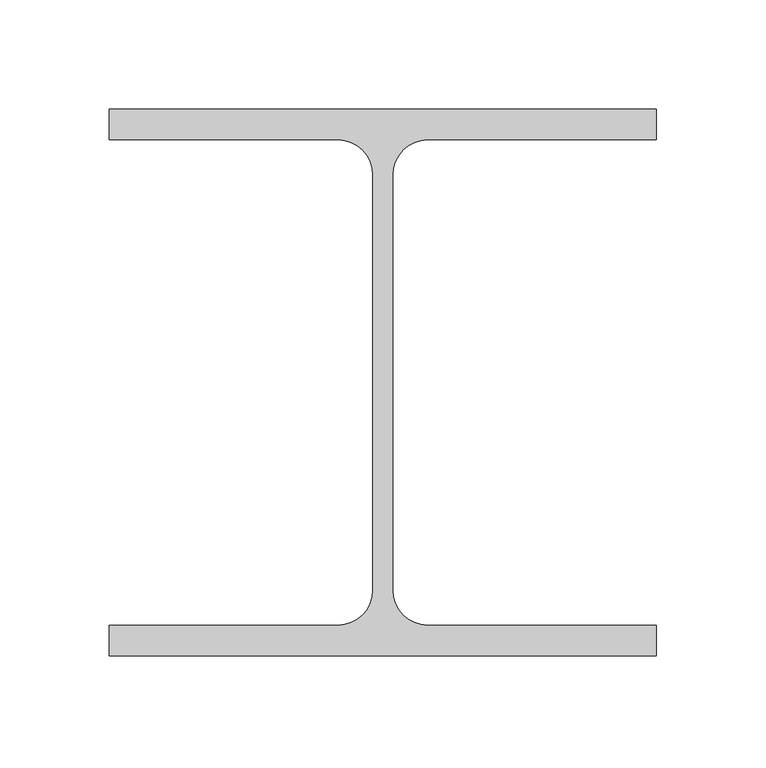
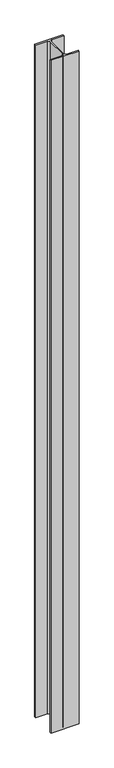
"""IFC4 building model written with IfcOpenShell, lengths in millimetres: column geometry, 0912_Steel Column_H_KSD3502 : H_SC_ASC_H-250x250x9x14."""

from ifc_helpers import new_model, si_unit, point, frame, frame_2d, origin, place, context, project, spatial, polyline, circle_curve, trimmed, segment, composite_curve, outline, extrude, source, transform, mapped, element, save


def column_a4b71116(model_context):
    return source(origin(), model_context, "Body", "SweptSolid", [
        extrude(outline(composite_curve([segment(polyline([(125.0, 125.0), (125.0, 111.0), (20.5, 111.0)]), True, "CONTINUOUS"), segment(trimmed(circle_curve(frame_2d((20.5, 95.0)), 16.0), [point((20.5, 111.0))], [point((4.5, 95.0))], True, "CARTESIAN"), True, "CONTINUOUS"), segment(polyline([(4.5, 95.0), (4.5, -95.0)]), True, "CONTINUOUS"), segment(trimmed(circle_curve(frame_2d((20.5, -95.0)), 16.0), [point((4.5, -95.0))], [point((20.5, -111.0))], True, "CARTESIAN"), True, "CONTINUOUS"), segment(polyline([(20.5, -111.0), (125.0, -111.0), (125.0, -125.0), (-125.0, -125.0), (-125.0, -111.0), (-20.5, -111.0)]), True, "CONTINUOUS"), segment(trimmed(circle_curve(frame_2d((-20.5, -95.0)), 16.0), [point((-20.5, -111.0))], [point((-4.5, -95.0))], True, "CARTESIAN"), True, "CONTINUOUS"), segment(polyline([(-4.5, -95.0), (-4.5, 95.0)]), True, "CONTINUOUS"), segment(trimmed(circle_curve(frame_2d((-20.5, 95.0)), 16.0), [point((-4.5, 95.0))], [point((-20.5, 111.0))], True, "CARTESIAN"), True, "CONTINUOUS"), segment(polyline([(-20.5, 111.0), (-125.0, 111.0), (-125.0, 125.0), (125.0, 125.0)]), True, "CONTINUOUS")], self_intersect=False)), frame((0.0, 0.0, 599.9720055), z_axis=(0.0, 0.0, 1.0), x_axis=(1.0, 0.0, 0.0)), (0.0, 0.0, 1.0), 6300.0),
    ])


if __name__ == "__main__":
    model = new_model("IFC4")
    model_context = context("Model", 3, world=origin())
    ifc_project = project(units=[si_unit("LENGTHUNIT", "METRE", prefix="MILLI")], contexts=[model_context])
    site = spatial("IfcSite", under=ifc_project)
    building = spatial("IfcBuilding", under=site)
    placement = place(None, origin())
    column_shape = column_a4b71116(model_context)
    element("IfcColumn", 1, ObjectType="0912_Steel Column_H_KSD3502 : H_SC_ASC_H-250x250x9x14", at=placement, inside=building, context=model_context, shape_type="MappedRepresentation", body=[
        mapped(column_shape, transform((0.0, 0.0, 0.0), x_axis=(1.0, 0.0, 0.0), y_axis=(0.0, 1.0, 0.0), z_axis=(0.0, 0.0, 1.0))),
    ])
    save(model, "model.ifc")

# Revit data of these elements
# Type "0912_Steel Column_H_KSD3502 : H_SC_ASC_H-250x250x9x14"
#   H_WM Code_1 = "S01AA002-00001 | Main Steel Structure Fabrication Work | Shelter/Building | Medium Steel - Standard (90KG/M>Weight≥30KG/M) | Material: (   )"
#   H_WM Code_2 = "S03AA028-00001 | Main Steel Structure Erection Work | Shelter/Building | Medium Steel (90KG/M>Weight≥30KG/M) | Material: (   )"
#   H_WM Code_3 = "S01AA010-00001 | Main Steel Structure Fabrication Work | Shelter/Building | Steel Painting/Coating | for Non-Fireproofed Steel Surface, Surface Preparation, Primer, Second & Final Coat | Material: (   )"
#   H_Q'ty Cal Type Tag = "SC-Q2"
#   Width = 25.0 cm
#   Web Thickness = 0.9 cm
#   Web Fillet = 1.6 cm
#   Warping Constant = 507646.0 cm⁶
#   Torsional Moment of Inertia = 51.4681 cm⁴
#   Section Area = 92.18 cm²
#   Plastic Modulus weak axis = 444.0 cm³
#   Plastic Modulus strong axis = 960.0 cm³
#   Perimeter = 1.46 m²/m
#   Nominal Weight = 72.40 kgf/m
#   Moment of Inertia weak axis = 3650.00 cm⁴
#   Moment of Inertia strong axis = 10800.00 cm⁴
#   Height = 25.0 cm
#   Flange Thickness = 1.4 cm
#   Elastic Modulus weak axis = 292.0 cm³
#   Elastic Modulus strong axis = 867.0 cm³
#   Centroid Vertical = 12.5 cm
#   Centroid Horizontal = 12.5 cm
#   Structural Material [instance default] = Steel, 45-345
#   Section Name Key = ""
#   Bolt Spacing = 0
#   Assembly Code = ""
# Element 1 (IfcColumn, "0912_Steel Column_H_KSD3502 : H_SC_ASC_H-250x250x9x14")
#   Structural Material = A03AD029-00005_Anchor Bolt (Installation only)_M24
#   Materials on its faces: "A03AD029-00005_Anchor Bolt (Installation only)_M24"
# Materials
#   "Steel, 45-345": class "Metal", colour RGB 189 187 185, transparency 0, Description = "Steel 345 MPa", Cost = 0
#   "A03AD029-00005_Anchor Bolt (Installation only)_M24": class "Unassigned", colour RGB 84 83 81, transparency 0, Cost = 0
